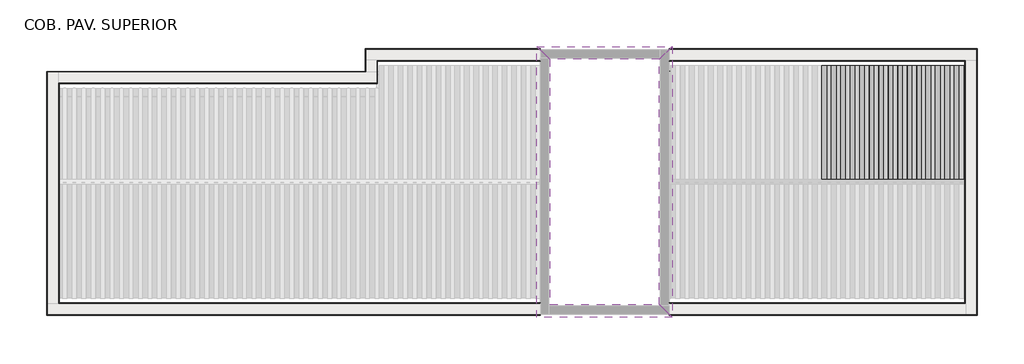
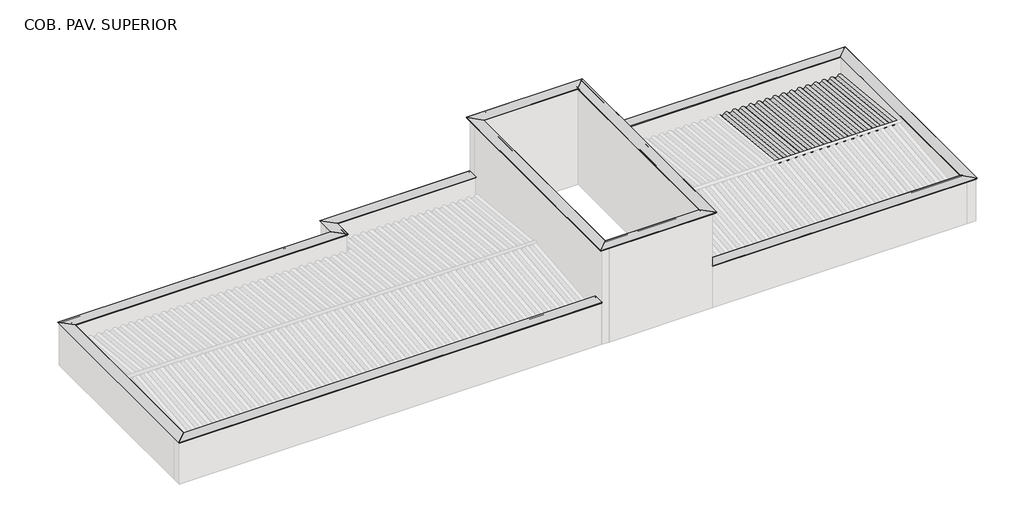
# One storey, part 7 of 7: 23 beams, 8 columns, 4 proxies.
# Revit data of these elements (continued)
# Elements 9, 10, 11, 12, 13, 14, 15, 16, 17, 18, 19, 20, 21, 22, 23 (IfcBeam, "Telha Ondulada : Fibrocimento") (continued)
#   Materials on its faces: ".TELHA DE FIBROCIMENTO"
# Element 24 (IfcBuildingElementProxy, ".CC_RUFO_PINGADEIRA_27 cm")
#   Uso = "RUFOS COB. PAV. SUPERIOR"
#   Phase Created = CC_PE
#   Materials on its faces: ".ALUMÍNIO COM PINTURA LÁTEX BRANCA"
# Elements 25, 26, 27 (IfcBuildingElementProxy, ".CC_RUFO_PINGADEIRA_27 cm")
#   Uso = "RUFOS COB. CAIXA D'ÁGUA"
#   Phase Created = CC_PE
#   Materials on its faces: ".ALUMÍNIO COM PINTURA LÁTEX BRANCA"
# Elements 28, 29, 30, 31, 32, 33, 34, 35 (IfcColumn, "Madeira de lei-Coluna : Pontalete 6X16cm")
#   Comments = ""
#   Structural Material = .MADEIRAMENTO
#   Phase Created = CC_PE
#   Materials on its faces: ".MADEIRAMENTO"
# Materials
#   ".TELHA DE FIBROCIMENTO": class "CC_TELHADO", colour RGB 77 77 76, transparency 0, Description = "TELHA ONDULADA FIBROCIMENTO", Cost = 0
#   ".MADEIRAMENTO": class ".CC_MADEIRAS", colour RGB 212 179 113, transparency 0, Cost = 0
#   ".ALUMÍNIO COM PINTURA LÁTEX BRANCA": class "Generic", colour RGB 250 250 250, transparency 0, Cost = 0
